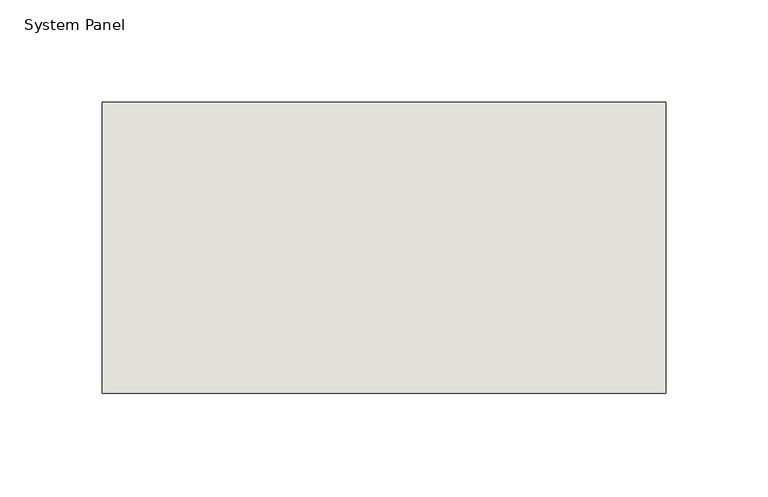
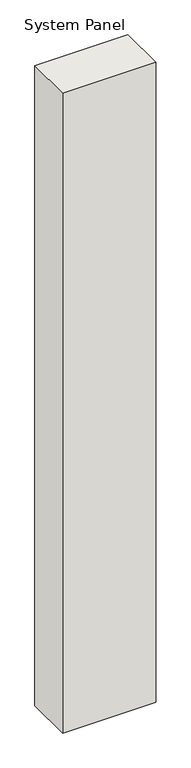
"""IFC4 building model written with IfcOpenShell, lengths in millimetres: wall geometry, System Panel : NLRS_21_CWP_hsb-vulling minerale wol 142 _gen_rsf."""

from ifc_helpers import new_model, si_unit, origin, origin_with_axes, place, context, project, spatial, polyline, outline, extrude, source, transform, mapped, element, save


def system_panel_e40bc043(model_context):
    return source(origin(), model_context, "Body", "SweptSolid", [
        extrude(outline(polyline([(137.422053, -71.0), (-137.422053, -71.0), (-137.422053, 71.0), (137.422053, 71.0), (137.422053, -71.0)])), origin_with_axes(), (0.0, 0.0, 1.0), 2000.0),
    ])


if __name__ == "__main__":
    model = new_model("IFC4")
    model_context = context("Model", 3, world=origin())
    ifc_project = project(units=[si_unit("LENGTHUNIT", "METRE", prefix="MILLI")], contexts=[model_context])
    site = spatial("IfcSite", under=ifc_project)
    building = spatial("IfcBuilding", under=site)
    placement = place(None, origin())
    system_panel_shape = system_panel_e40bc043(model_context)
    element("IfcWall", 1, ObjectType="System Panel : NLRS_21_CWP_hsb-vulling minerale wol 142 _gen_rsf", at=placement, inside=building, context=model_context, shape_type="MappedRepresentation", body=[
        mapped(system_panel_shape, transform((0.0, 0.0, 0.0), x_axis=(1.0, 0.0, 0.0), y_axis=(0.0, 1.0, 0.0), z_axis=(0.0, 0.0, 1.0))),
    ])
    save(model, "model.ifc")

# Revit data of these elements
# Type "System Panel : NLRS_21_CWP_hsb-vulling minerale wol 142 _gen_rsf"
#   Type IfcGUID = "07M7mRoiH1CR8m_RSKIwpC"
#   Assembly Code = "21.23"
#   IfcExportAs = "IfcWall"
# Element 1 (IfcWall, "System Panel : NLRS_21_CWP_hsb-vulling minerale wol 142 _gen_rsf")
#   Materials on its faces: "NLRS_m1_isolatie minerale wol_gen_rsf"
# Materials
#   "NLRS_m1_isolatie minerale wol_gen_rsf": class "M - Anorganische materialen", colour RGB 200 200 140, transparency 0, Keynote = "m1", Manufacturer = "Revit Standards Foundation", URL = "www.revitstandards.org", Description = "isolatie minerale wol", Cost = 0
